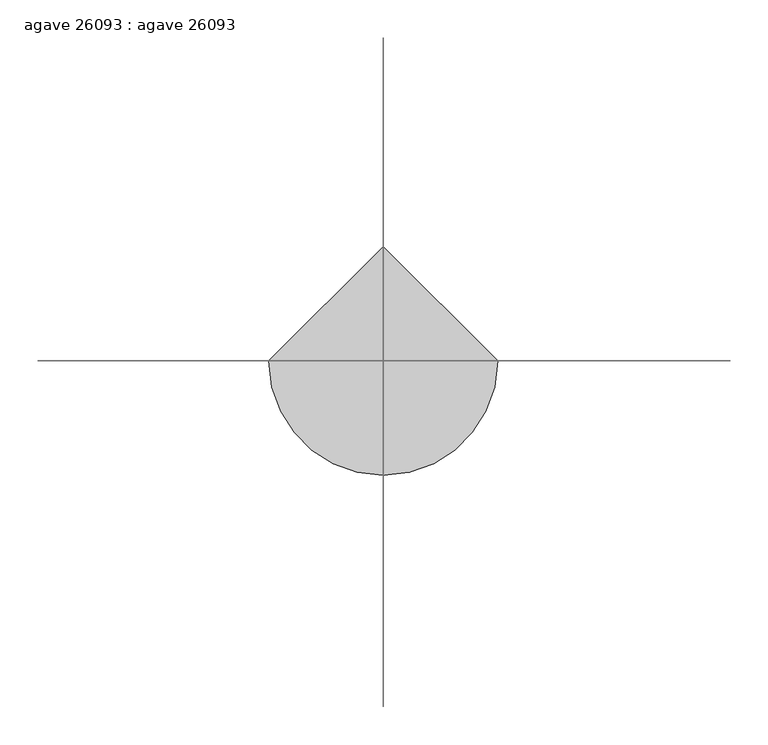
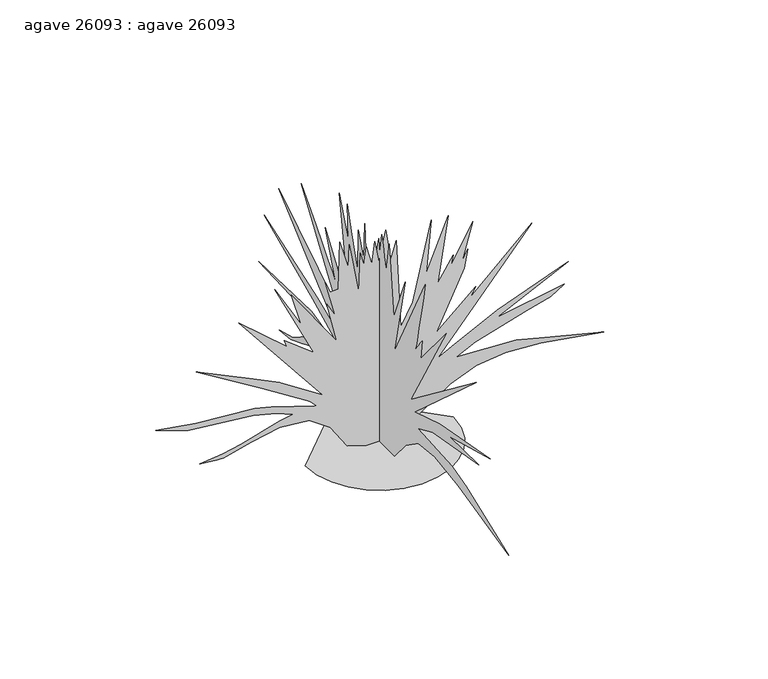
"""IFC4 building model written with IfcOpenShell, lengths in millimetres: proxy geometry, agave 26093 : agave 26093."""

import ifcopenshell
import ifcopenshell.guid

model = None  # the IFC model being written
_history = None  # IfcOwnerHistory: only IFC2X3 demands one
_inside = {}  # id of a spatial element -> (the spatial element, [elements in it])
_under = {}  # id of a project, library or spatial element -> (it, [spatial elements below it])
_declared = {}  # id of a project -> (the project, [libraries it declares])
_typed = {}  # id of a type object -> (the type object, [elements of that type])
_made_of = {}  # id of a material, layer set ... -> (it, [elements and type objects made of it])


def new_model(schema):
    """Start an empty IFC model of exactly this schema.

    Asked for "IFC4X3", IfcOpenShell would pick the latest addendum, in which some entities
    have other attributes; the version numbers below select the first issue.
    IFC2X3 requires an IfcOwnerHistory on every rooted entity: one is made here for all.
    """
    global model, _history
    if schema == "IFC4X3":
        model = ifcopenshell.file(schema_version=(4, 3, 0, 0))
    else:
        model = ifcopenshell.file(schema=schema)
    _inside.clear()
    _under.clear()
    _declared.clear()
    _typed.clear()
    _made_of.clear()
    _history = None
    if model.schema == "IFC2X3":
        org = make("IfcOrganization", Name="unknown")
        user = make(
            "IfcPersonAndOrganization",
            ThePerson=make("IfcPerson", FamilyName="unknown"),
            TheOrganization=org,
        )
        app = make(
            "IfcApplication",
            ApplicationDeveloper=org,
            Version="unknown",
            ApplicationFullName="unknown",
            ApplicationIdentifier="unknown",
        )
        _history = make(
            "IfcOwnerHistory",
            OwningUser=user,
            OwningApplication=app,
            ChangeAction="ADDED",
            CreationDate=0,
        )
    return model


def make(cls, **values):
    """One entity of the class cls with the attributes given. An attribute that is None is left unset."""
    return model.create_entity(
        cls, **{name: value for name, value in values.items() if value is not None}
    )


def rooted(cls, **values):
    """An entity with a GlobalId (a new one), such as an element, a storey or a relation."""
    return make(cls, GlobalId=ifcopenshell.guid.new(), OwnerHistory=_history, **values)


def si_unit(unit_type, name, prefix=None):
    """IfcSIUnit, for example si_unit("LENGTHUNIT", "METRE", prefix="MILLI")."""
    return make("IfcSIUnit", UnitType=unit_type, Prefix=prefix, Name=name)


def assignment(units):
    """IfcUnitAssignment: the units of a project."""
    return None if units is None else make("IfcUnitAssignment", Units=units)


def point(xyz):
    """IfcCartesianPoint."""
    return None if xyz is None else make("IfcCartesianPoint", Coordinates=xyz)


def direction(xyz):
    """IfcDirection."""
    return None if xyz is None else make("IfcDirection", DirectionRatios=xyz)


def frame(location, z_axis=None, x_axis=None):
    """IfcAxis2Placement3D, a coordinate frame: its origin and axes. An axis left out is left unset."""
    return make(
        "IfcAxis2Placement3D",
        Location=point(location),
        Axis=direction(z_axis),
        RefDirection=direction(x_axis),
    )


def origin():
    """The frame at (0, 0, 0) with its axes left unset."""
    return frame((0.0, 0.0, 0.0))


def place(relative_to, where):
    """IfcLocalPlacement: puts the frame where relative to a parent placement (None: the world)."""
    return make(
        "IfcLocalPlacement", PlacementRelTo=relative_to, RelativePlacement=where
    )


def context(
    kind, dimensions, precision=None, world=None, true_north=None, identifier=None
):
    """IfcGeometricRepresentationContext, for example the 3D "Model" context."""
    return make(
        "IfcGeometricRepresentationContext",
        ContextIdentifier=identifier,
        ContextType=kind,
        CoordinateSpaceDimension=dimensions,
        Precision=precision,
        WorldCoordinateSystem=world,
        TrueNorth=true_north,
    )


def project(units=None, contexts=None):
    """IfcProject with its units and contexts."""
    return rooted(
        "IfcProject",
        Name="project",
        RepresentationContexts=contexts,
        UnitsInContext=assignment(units),
    )


def spatial(cls, under=None, at=None, **own):
    """A site, building, storey or space (cls), placed at a placement, below another one or the project."""
    s = rooted(cls, ObjectPlacement=at, **own)
    if under is not None:
        _under.setdefault(under.id(), (under, []))[1].append(s)
    return s


def point_list(points):
    """IfcCartesianPointList2D or 3D."""
    cls = (
        "IfcCartesianPointList2D" if len(points[0]) == 2 else "IfcCartesianPointList3D"
    )
    return make(cls, CoordList=points)


def triangles(points, corners, closed=None, point_numbers=None):
    """IfcTriangulatedFaceSet: each triangle names its three corners, points numbered from 1."""
    return make(
        "IfcTriangulatedFaceSet",
        Coordinates=point_list(points),
        Closed=closed,
        CoordIndex=corners,
        PnIndex=point_numbers,
    )


def shape(context_of_items, identifier, shape_type, items):
    """IfcShapeRepresentation: the items that make up one representation, for example the "Body"."""
    return make(
        "IfcShapeRepresentation",
        ContextOfItems=context_of_items,
        RepresentationIdentifier=identifier,
        RepresentationType=shape_type,
        Items=items,
    )


def source(mapping_origin, context_of_items, identifier, shape_type, items):
    """IfcRepresentationMap: a shape defined once, which mapped items show again and again."""
    return make(
        "IfcRepresentationMap",
        MappingOrigin=mapping_origin,
        MappedRepresentation=shape(context_of_items, identifier, shape_type, items),
    )


def transform(
    local_origin,
    x_axis=None,
    y_axis=None,
    z_axis=None,
    scale=None,
    scale2=None,
    scale3=None,
    uniform=True,
):
    """IfcCartesianTransformationOperator3D, or its non-uniform kind. x_axis, y_axis, z_axis: its Axis1, 2, 3."""
    if uniform:
        return make(
            "IfcCartesianTransformationOperator3D",
            Axis1=direction(x_axis),
            Axis2=direction(y_axis),
            LocalOrigin=point(local_origin),
            Scale=scale,
            Axis3=direction(z_axis),
        )
    return make(
        "IfcCartesianTransformationOperator3DnonUniform",
        Axis1=direction(x_axis),
        Axis2=direction(y_axis),
        LocalOrigin=point(local_origin),
        Scale=scale,
        Axis3=direction(z_axis),
        Scale2=scale2,
        Scale3=scale3,
    )


def mapped(mapping_source, mapping_target):
    """IfcMappedItem: shows the shape of a source again, moved by a transform."""
    return make(
        "IfcMappedItem", MappingSource=mapping_source, MappingTarget=mapping_target
    )


def made_of(thing, what):
    """Note that an element or type object is made of a material, layer set ...; save() writes the relation."""
    if what is not None:
        _made_of.setdefault(what.id(), (what, []))[1].append(thing)
    return thing


def element(
    cls,
    number,
    at=None,
    inside=None,
    cuts=None,
    type_object=None,
    material=None,
    context=None,
    identifier="Body",
    shape_type=None,
    held_by="IfcProductDefinitionShape",
    body=None,
    shapes=None,
    **own,
):
    """One element of the class cls, such as IfcWall. Its Tag is "e" and its number.

    at: its placement. inside: the storey or other place that contains it. cuts: it is an
    opening in that element (IfcRelVoidsElement). A single representation is given by context,
    identifier, shape_type and body (its items); several are given by shapes. held_by: the class
    of the entity that holds the representations. save() writes the other relations.
    """
    e = rooted(cls, Tag="e%d" % number, ObjectPlacement=at, **own)
    if body is not None:
        shapes = [shape(context, identifier, shape_type, body)]
    if shapes is not None:
        e.Representation = make(held_by, Representations=shapes)
    if inside is not None:
        _inside.setdefault(inside.id(), (inside, []))[1].append(e)
    if cuts is not None:
        rooted(
            "IfcRelVoidsElement", RelatingBuildingElement=cuts, RelatedOpeningElement=e
        )
    if type_object is not None:
        _typed.setdefault(type_object.id(), (type_object, []))[1].append(e)
    return made_of(e, material)


def aggregate(whole, parts):
    """IfcRelAggregates: a whole, such as a stair, and the parts it consists of."""
    return rooted("IfcRelAggregates", RelatingObject=whole, RelatedObjects=parts)


def save(model, path):
    """Write the relations noted so far, then the file.

    IfcRelAggregates (storeys below a building ...), IfcRelContainedInSpatialStructure (elements
    in a storey), IfcRelDefinesByType, IfcRelAssociatesMaterial and IfcRelDeclares: one each for
    every whole, place, type object, material and project.
    """
    for whole, parts in _under.values():
        aggregate(whole, parts)
    for where, things in _inside.values():
        rooted(
            "IfcRelContainedInSpatialStructure",
            RelatedElements=things,
            RelatingStructure=where,
        )
    for kind, things in _typed.values():
        rooted("IfcRelDefinesByType", RelatedObjects=things, RelatingType=kind)
    for what, things in _made_of.values():
        rooted("IfcRelAssociatesMaterial", RelatedObjects=things, RelatingMaterial=what)
    for by, libraries in _declared.values():
        rooted("IfcRelDeclares", RelatingContext=by, RelatedDefinitions=libraries)
    model.write(path)


def agave_26093_agave_26093_93a2a214(model_context):
    return source(origin(), model_context, "Body", "Tessellation", [
        triangles([(-150.7087333, 0.0, 9.4e-06), (-146.7244834, -34.5323444, 9.4e-06), (-135.3772836, -66.2450299, 9.4e-06), (-117.5759356, -94.2289958, 9.4e-06), (-94.2289958, -117.5759356, 9.4e-06), (-66.2450299, -135.3772836, 9.4e-06), (-34.5323444, -146.7244834, 9.4e-06), (6.6e-06, -150.7087333, 9.4e-06), (34.5323444, -146.7244834, 9.4e-06), (66.2450299, -135.3772836, 9.4e-06), (94.2289958, -117.5759356, 9.4e-06), (117.5759356, -94.2289958, 9.4e-06), (135.3772836, -66.2450299, 9.4e-06), (146.7244834, -34.5323444, 9.4e-06), (150.7087333, 1.32e-05, 9.4e-06), (-1.98e-05, 150.7087333, 9.4e-06), (-24.9398476, 1.1e-06, 2.5e-06), (-65.4258802, 2.1e-06, 13.141818), (-99.6620581, 5e-07, 65.0964399), (-143.0435126, 6e-07, 95.6658721), (-202.3246234, 2.8e-06, 101.1403381), (-259.7355268, 6e-06, 89.1792132), (-316.7763402, 9.4e-06, 74.9889865), (-329.6211594, 9.9e-06, 75.5035945), (-365.3285002, 1.12e-05, 79.1975187), (-318.313056, 8.9e-06, 84.1103911), (-282.3389982, 6.9e-06, 91.7898278), (-203.1008479, 2e-06, 114.8573697), (-175.7107319, 5e-07, 119.829677), (-208.3624635, 1.2e-06, 133.0887423), (-256.7688111, 2.5e-06, 145.787731), (-389.2832517, 7.5e-06, 160.0767662), (-455.2115313, 9e-06, 182.6248811), (-373.9467241, 6.3e-06, 169.0808314), (-253.2813787, 1.6e-06, 159.2306877), (-220.3573709, 6e-07, 151.0805947), (-127.6907252, -1.6e-06, 121.0610699), (-140.4735387, -1.9e-06, 135.3043865), (-238.3492232, -1.3e-06, 197.06021), (-372.7148226, -4e-07, 279.8955245), (-256.342093, -2.1e-06, 224.048243), (-204.0302424, -2.9e-06, 198.6317166), (-115.3780683, -3.3e-06, 140.7615752), (-286.5249345, -8.6e-06, 355.0033673), (-188.0233888, -7.9e-06, 270.045399), (-192.9487059, -8.5e-06, 284.8205873), (-133.8471808, -8.3e-06, 238.0324729), (-212.6492294, -1.47e-05, 401.7927715), (-158.472758, -1.14e-05, 306.9846414), (-179.4046562, -1.47e-05, 378.3993593), (-87.0585669, -1.09e-05, 246.6514781), (-106.7590813, -1.52e-05, 332.8418567), (-89.5210982, -1.41e-05, 302.0595786), (-110.4530055, -1.79e-05, 380.860619), (-99.717687, -1.69e-05, 356.9287222), (-83.2732056, -1.76e-05, 356.9490335), (-80.9021112, -2.37e-05, 457.2003633), (-63.426897, -2.09e-05, 396.9718449), (-61.2016014, -2.38e-05, 444.8864347), (-41.5013458, -1.82e-05, 335.3031163), (-39.0385601, -2.33e-05, 419.0317629), (-31.650966, -2.19e-05, 390.7107445), (-26.7259009, -2.44e-05, 428.8818884), (-15.6443803, -2.24e-05, 387.0175833), (-9.4879996, -2.54e-05, 433.8069511), (-0.8690236, -2.3e-05, 387.0175833), (12.6750416, -2.74e-05, 451.043399), (23.7565623, -2.39e-05, 383.3244221), (34.8381601, -2.66e-05, 420.261121), (43.4571494, -1.56e-05, 230.6448788), (68.0824677, -1.94e-05, 276.2023633), (105.4982208, -3.08e-05, 439.9537416), (95.1708261, -2.38e-05, 329.146152), (140.4829403, -3.22e-05, 436.9539974), (118.5650104, -2.3e-05, 299.5957755), (150.578436, -2.74e-05, 348.8489465), (145.6533642, -2.58e-05, 326.6848924), (189.9794467, -3.25e-05, 406.7178343), (167.81641, -2.69e-05, 327.9167939), (180.1290669, -2.88e-05, 351.3102061), (173.4681726, -2.62e-05, 313.009528), (116.102479, -1.66e-05, 193.7063995), (196.1359024, -2.44e-05, 265.1203362), (183.8229911, -2.26e-05, 244.1889286), (310.6447741, -3.51e-05, 361.1603316), (118.5650104, -1.34e-05, 138.2987895), (158.4747927, -1.63e-05, 158.0775423), (240.4617396, -2.24e-05, 198.6317166), (384.5207517, -3.19e-05, 252.8079337), (239.2306011, -2.13e-05, 182.6248811), (376.7864491, -2.88e-05, 206.3655105), (349.174072, -2.66e-05, 189.8819236), (300.4111145, -2.36e-05, 176.0696308), (195.4584909, -1.73e-05, 146.0828801), (156.7348917, -1.44e-05, 127.2172711), (278.6305944, -1.94e-05, 121.0610699), (336.3953462, -2.1e-05, 106.1004551), (457.1673348, -2.45e-05, 75.5035945), (329.0750444, -2.01e-05, 96.2046111), (257.431743, -1.73e-05, 101.1027496), (197.4574787, -1.42e-05, 94.105802), (144.7537007, -1.07e-05, 73.3684686), (86.5066293, -5.8e-06, 34.1325482), (33.0588878, -1.4e-06, 0.0), (9e-07, 20.0836192, 9.1e-06), (2.1e-06, 47.8000438, 9.9e-06), (3.7e-06, 68.4088604, 20.0829062), (6.2e-06, 99.6950775, 59.1195655), (8.3e-06, 132.7178983, 80.7177112), (1.03e-05, 174.2748821, 84.8467378), (1.15e-05, 208.5839434, 72.8693576), (1.35e-05, 272.2425033, 45.8366235), (1.48e-05, 311.9833551, 30.2844433), (1.65e-05, 353.3269798, 25.0212039), (1.48e-05, 305.3793614, 38.860505), (1.34e-05, 249.7515432, 74.8251566), (1.18e-05, 199.8564965, 97.660536), (1.01e-05, 161.2479701, 96.4354927), (1.17e-05, 188.527337, 110.366392), (1.51e-05, 256.1160167, 122.0234748), (2.29e-05, 425.717038, 129.5510222), (1.47e-05, 238.8183625, 134.6051196), (1.09e-05, 164.9452008, 118.743824), (8.2e-06, 119.3844099, 96.4354927), (1.1e-05, 159.9457058, 127.6671074), (1.54e-05, 233.8196305, 165.2718342), (2.53e-05, 406.273312, 240.4952587), (1.5e-05, 217.8867004, 177.6998184), (1.1e-05, 147.7036569, 148.1491784), (2.57e-05, 354.5588814, 329.146152), (1.25e-05, 146.2032761, 198.5547591), (2.38e-05, 274.5259576, 388.2494848), (2.18e-05, 248.7817623, 359.4966614), (1.99e-05, 223.9913424, 331.6328098), (1.81e-05, 201.1074557, 305.5495545), (1.65e-05, 181.0833509, 282.1358129), (1.52e-05, 164.872549, 262.2780679), (1.42e-05, 153.4283166, 246.8711776), (1.37e-05, 147.7036569, 236.8013344), (1.88e-05, 190.798601, 345.1532418), (1.51e-05, 148.9134577, 283.7461616), (1.48e-05, 144.9251474, 278.3410409), (1.44e-05, 140.1001603, 272.7403471), (1.4e-05, 134.5776867, 266.9770725), (1.35e-05, 128.4971803, 261.086807), (1.31e-05, 121.9980766, 255.0974924), (1.26e-05, 115.2200837, 249.0439011), (1.21e-05, 108.3028915, 242.95779), (1.97e-05, 140.3160628, 449.8114975), (1.58e-05, 109.53403, 367.3172959), (1.82e-05, 113.2279542, 442.4251751), (1.61e-05, 98.452766, 393.1745476), (1.29e-05, 75.0583319, 320.5279281), (1.55e-05, 73.826939, 410.4109955), (1.32e-05, 55.357822, 358.699072), (1.53e-05, 51.6638932, 437.5001123), (1.36e-05, 47.2595336, 384.1829453), (1.1e-05, 27.0383205, 327.9167939), (1.31e-05, 1.1814591, 436.2682108), (1.2e-05, -1.2811313, 405.4859327), (1.3e-05, -8.5500533, 450.4566616), (1.25e-05, -11.9783704, 436.1437634), (1.19e-05, -15.2441015, 422.2677209), (1.14e-05, -18.1847128, 409.2629188), (1.09e-05, -20.6375916, 397.5687561), (1.05e-05, -22.4401819, 387.6195451), (1.03e-05, -23.4298925, 379.852214), (1.01e-05, -23.4441676, 374.7036547), (1.18e-05, -34.5257405, 446.1183363), (6.6e-06, -50.5323262, 298.3664174), (7.8e-06, -92.3958773, 399.3315119), (4.4e-06, -52.9948575, 225.7198161), (5.7e-06, -162.5786665, 436.2682108), (5.1e-06, -155.9520543, 404.0000133), (4.4e-06, -149.5159464, 372.9078704), (3.8e-06, -143.4613468, 344.1651844), (3.3e-06, -137.9787509, 318.9480463), (2.9e-06, -133.2591716, 298.4324563), (2.7e-06, -129.4933677, 283.7918891), (2.6e-06, -126.87158, 276.2023633), (2.5e-06, -126.0089964, 274.2135312), (2.5e-06, -127.1682462, 275.2524031), (2.5e-06, -130.0120315, 278.8160301), (2.5e-06, -134.204054, 284.398956), (2.5e-06, -139.4067433, 291.4957067), (2.4e-06, -145.2835467, 299.6034059), (2.4e-06, -151.4971481, 308.2165429), (1.4e-06, -145.3409469, 266.3522378), (6e-07, -236.4556433, 375.9355562), (-2e-07, -110.8649898, 157.9992949), (-5.3e-06, -341.1146439, 334.0712148), (-1.4e-06, -124.4090487, 138.2990438), (-4.6e-06, -213.0612137, 166.6183), (-1.15e-05, -391.2898516, 199.4396978), (-6.2e-06, -246.3057688, 160.4618262), (-1.09e-05, -351.4651749, 162.9246119), (-4.5e-06, -189.3266705, 133.5012353), (-2.8e-06, -135.490567, 109.9795515), (-8.4e-06, -257.3885589, 102.5916939), (-1.11e-05, -306.6392046, 89.0476442), (-1.94e-05, -455.623025, 31.1775097), (-1.03e-05, -278.0057598, 72.8693576), (-6.2e-06, -195.1343828, 85.0082832), (-3.8e-06, -137.6096873, 78.9734862), (-2.8e-06, -94.1832773, 48.8668437), (-2.4e-06, -52.6021717, 6.9e-06), (-9e-07, -19.1255291, 7.9e-06)], [[15, 16, 1], [14, 15, 1], [14, 1, 2], [13, 14, 2], [13, 2, 3], [13, 3, 4], [12, 13, 4], [11, 12, 4], [11, 4, 5], [11, 5, 6], [11, 6, 7], [11, 7, 8], [11, 8, 9], [11, 9, 10], [47, 48, 49], [97, 98, 99], [88, 89, 90], [39, 40, 41], [84, 85, 86], [71, 72, 73], [53, 54, 55], [32, 33, 34], [43, 44, 45], [24, 25, 26], [58, 59, 60], [77, 78, 79], [73, 74, 75], [60, 61, 62], [51, 52, 53], [56, 57, 58], [82, 83, 84], [79, 80, 81], [64, 65, 66], [49, 50, 51], [68, 69, 70], [75, 76, 77], [90, 91, 92], [90, 92, 93], [66, 67, 68], [82, 84, 86], [90, 93, 94], [62, 63, 64], [47, 49, 51], [39, 41, 42], [45, 46, 47], [43, 45, 47], [38, 39, 42], [38, 42, 43], [31, 32, 34], [31, 34, 35], [23, 24, 26], [56, 58, 60], [87, 88, 90], [87, 90, 94], [87, 94, 95], [37, 38, 43], [86, 87, 95], [71, 73, 75], [96, 97, 99], [96, 99, 100], [95, 96, 100], [95, 100, 101], [95, 101, 102], [53, 55, 56], [53, 56, 60], [22, 23, 26], [22, 26, 27], [22, 27, 28], [21, 22, 28], [60, 62, 64], [43, 47, 51], [30, 31, 35], [30, 35, 36], [30, 36, 37], [29, 30, 37], [86, 95, 102], [21, 28, 29], [20, 21, 29], [20, 29, 37], [19, 20, 37], [86, 102, 103], [66, 68, 70], [64, 66, 70], [60, 64, 70], [53, 60, 70], [51, 53, 70], [43, 51, 70], [77, 79, 81], [77, 81, 82], [75, 77, 82], [71, 75, 82], [70, 71, 82], [70, 82, 86], [43, 70, 86], [43, 86, 103], [43, 103, 104], [43, 104, 17], [43, 17, 18], [43, 18, 19], [43, 19, 37], [120, 121, 122], [193, 194, 195], [190, 191, 192], [126, 127, 128], [155, 156, 157], [131, 132, 133], [200, 201, 202], [113, 114, 115], [195, 196, 197], [129, 130, 131], [131, 133, 134], [170, 171, 172], [188, 189, 190], [131, 134, 135], [148, 149, 150], [139, 140, 141], [131, 135, 136], [150, 151, 152], [168, 169, 170], [172, 173, 174], [131, 136, 137], [158, 159, 160], [172, 174, 175], [131, 137, 138], [153, 154, 155], [131, 138, 139], [172, 175, 176], [160, 161, 162], [172, 176, 177], [186, 187, 188], [172, 177, 178], [112, 113, 115], [112, 115, 116], [111, 112, 116], [111, 116, 117], [160, 162, 163], [172, 178, 179], [172, 179, 180], [172, 180, 181], [139, 141, 142], [193, 195, 197], [185, 186, 188], [192, 193, 197], [192, 197, 198], [155, 157, 158], [150, 152, 153], [148, 150, 153], [139, 142, 143], [199, 200, 202], [119, 120, 122], [119, 122, 123], [118, 119, 123], [199, 202, 203], [198, 199, 203], [198, 203, 204], [184, 185, 188], [110, 111, 117], [110, 117, 118], [109, 110, 118], [160, 163, 164], [118, 123, 124], [109, 118, 124], [139, 143, 144], [125, 126, 128], [125, 128, 129], [183, 184, 188], [139, 144, 145], [153, 155, 158], [108, 109, 124], [139, 145, 146], [160, 164, 165], [158, 160, 165], [158, 165, 166], [158, 166, 167], [158, 167, 168], [158, 168, 170], [182, 183, 188], [124, 125, 129], [182, 188, 190], [181, 182, 190], [172, 181, 190], [139, 146, 147], [131, 139, 147], [131, 147, 148], [158, 170, 172], [153, 158, 172], [148, 153, 172], [198, 204, 205], [131, 148, 172], [129, 131, 172], [124, 129, 172], [124, 172, 190], [108, 124, 190], [107, 108, 190], [106, 107, 190], [105, 106, 190], [207, 105, 190], [206, 207, 190], [205, 206, 190], [198, 205, 190], [192, 198, 190]], closed=False),
    ])


if __name__ == "__main__":
    model = new_model("IFC4")
    model_context = context("Model", 3, world=origin())
    ifc_project = project(units=[si_unit("LENGTHUNIT", "METRE", prefix="MILLI")], contexts=[model_context])
    site = spatial("IfcSite", under=ifc_project)
    building = spatial("IfcBuilding", under=site)
    placement = place(None, origin())
    agave_26093_agave_26093_shape = agave_26093_agave_26093_93a2a214(model_context)
    element("IfcBuildingElementProxy", 1, Name="agave 26093 : agave 26093", ObjectType="agave 26093 : agave 26093", at=placement, inside=building, context=model_context, shape_type="MappedRepresentation", body=[
        mapped(agave_26093_agave_26093_shape, transform((0.0, 0.0, 0.0), x_axis=(1.0, 0.0, 0.0), y_axis=(0.0, 1.0, 0.0), z_axis=(0.0, 0.0, 1.0))),
    ])
    save(model, "model.ifc")

# Revit data of these elements
# Type "agave 26093 : agave 26093"
#   built-in parameter 1005195 = "RPC-16-G1GJ-63FX-7K5P-N000-ST1L-LVER-AU"
#   Height = 0
